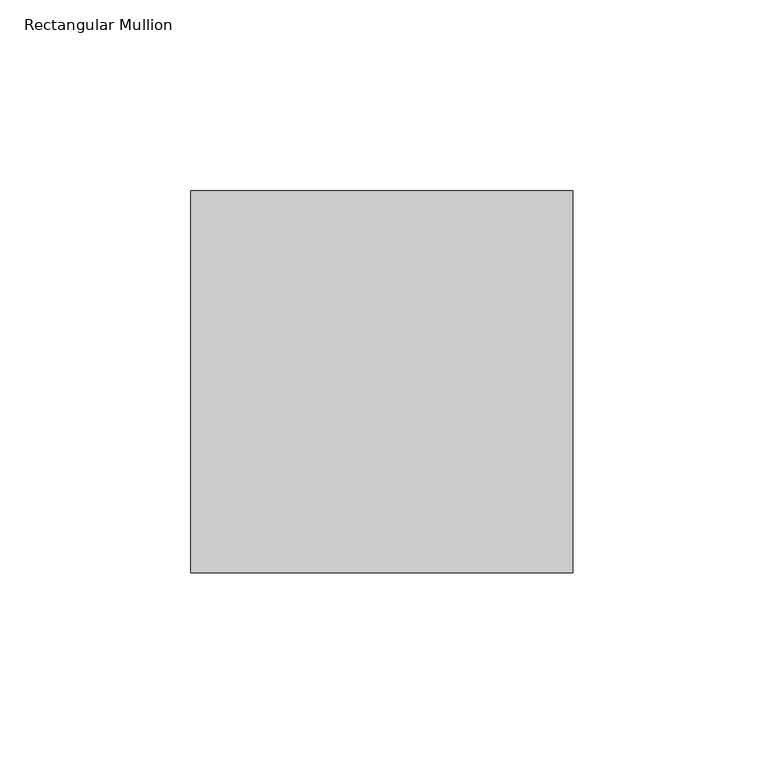
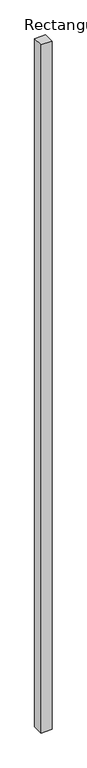
"""IFC4 building model written with IfcOpenShell, lengths in millimetres: member geometry, Rectangular Mullion : 알루미늄_Rectangular Cap_100 x100."""

import ifcopenshell
import ifcopenshell.guid

model = None  # the IFC model being written
_history = None  # IfcOwnerHistory: only IFC2X3 demands one
_inside = {}  # id of a spatial element -> (the spatial element, [elements in it])
_under = {}  # id of a project, library or spatial element -> (it, [spatial elements below it])
_declared = {}  # id of a project -> (the project, [libraries it declares])
_typed = {}  # id of a type object -> (the type object, [elements of that type])
_made_of = {}  # id of a material, layer set ... -> (it, [elements and type objects made of it])


def new_model(schema):
    """Start an empty IFC model of exactly this schema.

    Asked for "IFC4X3", IfcOpenShell would pick the latest addendum, in which some entities
    have other attributes; the version numbers below select the first issue.
    IFC2X3 requires an IfcOwnerHistory on every rooted entity: one is made here for all.
    """
    global model, _history
    if schema == "IFC4X3":
        model = ifcopenshell.file(schema_version=(4, 3, 0, 0))
    else:
        model = ifcopenshell.file(schema=schema)
    _inside.clear()
    _under.clear()
    _declared.clear()
    _typed.clear()
    _made_of.clear()
    _history = None
    if model.schema == "IFC2X3":
        org = make("IfcOrganization", Name="unknown")
        user = make(
            "IfcPersonAndOrganization",
            ThePerson=make("IfcPerson", FamilyName="unknown"),
            TheOrganization=org,
        )
        app = make(
            "IfcApplication",
            ApplicationDeveloper=org,
            Version="unknown",
            ApplicationFullName="unknown",
            ApplicationIdentifier="unknown",
        )
        _history = make(
            "IfcOwnerHistory",
            OwningUser=user,
            OwningApplication=app,
            ChangeAction="ADDED",
            CreationDate=0,
        )
    return model


def make(cls, **values):
    """One entity of the class cls with the attributes given. An attribute that is None is left unset."""
    return model.create_entity(
        cls, **{name: value for name, value in values.items() if value is not None}
    )


def rooted(cls, **values):
    """An entity with a GlobalId (a new one), such as an element, a storey or a relation."""
    return make(cls, GlobalId=ifcopenshell.guid.new(), OwnerHistory=_history, **values)


def si_unit(unit_type, name, prefix=None):
    """IfcSIUnit, for example si_unit("LENGTHUNIT", "METRE", prefix="MILLI")."""
    return make("IfcSIUnit", UnitType=unit_type, Prefix=prefix, Name=name)


def assignment(units):
    """IfcUnitAssignment: the units of a project."""
    return None if units is None else make("IfcUnitAssignment", Units=units)


def point(xyz):
    """IfcCartesianPoint."""
    return None if xyz is None else make("IfcCartesianPoint", Coordinates=xyz)


def direction(xyz):
    """IfcDirection."""
    return None if xyz is None else make("IfcDirection", DirectionRatios=xyz)


def frame(location, z_axis=None, x_axis=None):
    """IfcAxis2Placement3D, a coordinate frame: its origin and axes. An axis left out is left unset."""
    return make(
        "IfcAxis2Placement3D",
        Location=point(location),
        Axis=direction(z_axis),
        RefDirection=direction(x_axis),
    )


def origin():
    """The frame at (0, 0, 0) with its axes left unset."""
    return frame((0.0, 0.0, 0.0))


def place(relative_to, where):
    """IfcLocalPlacement: puts the frame where relative to a parent placement (None: the world)."""
    return make(
        "IfcLocalPlacement", PlacementRelTo=relative_to, RelativePlacement=where
    )


def context(
    kind, dimensions, precision=None, world=None, true_north=None, identifier=None
):
    """IfcGeometricRepresentationContext, for example the 3D "Model" context."""
    return make(
        "IfcGeometricRepresentationContext",
        ContextIdentifier=identifier,
        ContextType=kind,
        CoordinateSpaceDimension=dimensions,
        Precision=precision,
        WorldCoordinateSystem=world,
        TrueNorth=true_north,
    )


def project(units=None, contexts=None):
    """IfcProject with its units and contexts."""
    return rooted(
        "IfcProject",
        Name="project",
        RepresentationContexts=contexts,
        UnitsInContext=assignment(units),
    )


def spatial(cls, under=None, at=None, **own):
    """A site, building, storey or space (cls), placed at a placement, below another one or the project."""
    s = rooted(cls, ObjectPlacement=at, **own)
    if under is not None:
        _under.setdefault(under.id(), (under, []))[1].append(s)
    return s


def polyline(points):
    """IfcPolyline through the points."""
    return make("IfcPolyline", Points=[point(p) for p in points])


def outline(outer, holes=None, kind="AREA"):
    """IfcArbitraryClosedProfileDef: a profile drawn as a closed curve; with holes, ...WithVoids."""
    if holes is None:
        return make("IfcArbitraryClosedProfileDef", ProfileType=kind, OuterCurve=outer)
    return make(
        "IfcArbitraryProfileDefWithVoids",
        ProfileType=kind,
        OuterCurve=outer,
        InnerCurves=holes,
    )


def extrude(swept, where, along, depth):
    """IfcExtrudedAreaSolid: the profile swept, set in the frame where, extruded along a direction by depth."""
    return make(
        "IfcExtrudedAreaSolid",
        SweptArea=swept,
        Position=where,
        ExtrudedDirection=direction(along),
        Depth=depth,
    )


def shape(context_of_items, identifier, shape_type, items):
    """IfcShapeRepresentation: the items that make up one representation, for example the "Body"."""
    return make(
        "IfcShapeRepresentation",
        ContextOfItems=context_of_items,
        RepresentationIdentifier=identifier,
        RepresentationType=shape_type,
        Items=items,
    )


def source(mapping_origin, context_of_items, identifier, shape_type, items):
    """IfcRepresentationMap: a shape defined once, which mapped items show again and again."""
    return make(
        "IfcRepresentationMap",
        MappingOrigin=mapping_origin,
        MappedRepresentation=shape(context_of_items, identifier, shape_type, items),
    )


def transform(
    local_origin,
    x_axis=None,
    y_axis=None,
    z_axis=None,
    scale=None,
    scale2=None,
    scale3=None,
    uniform=True,
):
    """IfcCartesianTransformationOperator3D, or its non-uniform kind. x_axis, y_axis, z_axis: its Axis1, 2, 3."""
    if uniform:
        return make(
            "IfcCartesianTransformationOperator3D",
            Axis1=direction(x_axis),
            Axis2=direction(y_axis),
            LocalOrigin=point(local_origin),
            Scale=scale,
            Axis3=direction(z_axis),
        )
    return make(
        "IfcCartesianTransformationOperator3DnonUniform",
        Axis1=direction(x_axis),
        Axis2=direction(y_axis),
        LocalOrigin=point(local_origin),
        Scale=scale,
        Axis3=direction(z_axis),
        Scale2=scale2,
        Scale3=scale3,
    )


def mapped(mapping_source, mapping_target):
    """IfcMappedItem: shows the shape of a source again, moved by a transform."""
    return make(
        "IfcMappedItem", MappingSource=mapping_source, MappingTarget=mapping_target
    )


def made_of(thing, what):
    """Note that an element or type object is made of a material, layer set ...; save() writes the relation."""
    if what is not None:
        _made_of.setdefault(what.id(), (what, []))[1].append(thing)
    return thing


def element(
    cls,
    number,
    at=None,
    inside=None,
    cuts=None,
    type_object=None,
    material=None,
    context=None,
    identifier="Body",
    shape_type=None,
    held_by="IfcProductDefinitionShape",
    body=None,
    shapes=None,
    **own,
):
    """One element of the class cls, such as IfcWall. Its Tag is "e" and its number.

    at: its placement. inside: the storey or other place that contains it. cuts: it is an
    opening in that element (IfcRelVoidsElement). A single representation is given by context,
    identifier, shape_type and body (its items); several are given by shapes. held_by: the class
    of the entity that holds the representations. save() writes the other relations.
    """
    e = rooted(cls, Tag="e%d" % number, ObjectPlacement=at, **own)
    if body is not None:
        shapes = [shape(context, identifier, shape_type, body)]
    if shapes is not None:
        e.Representation = make(held_by, Representations=shapes)
    if inside is not None:
        _inside.setdefault(inside.id(), (inside, []))[1].append(e)
    if cuts is not None:
        rooted(
            "IfcRelVoidsElement", RelatingBuildingElement=cuts, RelatedOpeningElement=e
        )
    if type_object is not None:
        _typed.setdefault(type_object.id(), (type_object, []))[1].append(e)
    return made_of(e, material)


def aggregate(whole, parts):
    """IfcRelAggregates: a whole, such as a stair, and the parts it consists of."""
    return rooted("IfcRelAggregates", RelatingObject=whole, RelatedObjects=parts)


def save(model, path):
    """Write the relations noted so far, then the file.

    IfcRelAggregates (storeys below a building ...), IfcRelContainedInSpatialStructure (elements
    in a storey), IfcRelDefinesByType, IfcRelAssociatesMaterial and IfcRelDeclares: one each for
    every whole, place, type object, material and project.
    """
    for whole, parts in _under.values():
        aggregate(whole, parts)
    for where, things in _inside.values():
        rooted(
            "IfcRelContainedInSpatialStructure",
            RelatedElements=things,
            RelatingStructure=where,
        )
    for kind, things in _typed.values():
        rooted("IfcRelDefinesByType", RelatedObjects=things, RelatingType=kind)
    for what, things in _made_of.values():
        rooted("IfcRelAssociatesMaterial", RelatedObjects=things, RelatingMaterial=what)
    for by, libraries in _declared.values():
        rooted("IfcRelDeclares", RelatingContext=by, RelatedDefinitions=libraries)
    model.write(path)


def rectangular_mullion_46d195e2(model_context):
    return source(origin(), model_context, "Body", "SweptSolid", [
        extrude(outline(polyline([(0.0, 50.0), (0.0, -50.0), (-100.0, -50.0), (-100.0, 50.0), (0.0, 50.0)])), frame((0.0, 0.0, -6569.0), z_axis=(0.0, 0.0, 1.0), x_axis=(1.0, 0.0, 0.0)), (0.0, 0.0, 1.0), 6569.0),
    ])


if __name__ == "__main__":
    model = new_model("IFC4")
    model_context = context("Model", 3, world=origin())
    ifc_project = project(units=[si_unit("LENGTHUNIT", "METRE", prefix="MILLI")], contexts=[model_context])
    site = spatial("IfcSite", under=ifc_project)
    building = spatial("IfcBuilding", under=site)
    placement = place(None, origin())
    rectangular_mullion_shape = rectangular_mullion_46d195e2(model_context)
    element("IfcMember", 1, ObjectType="Rectangular Mullion : 알루미늄_Rectangular Cap_100 x100", at=placement, inside=building, context=model_context, shape_type="MappedRepresentation", body=[
        mapped(rectangular_mullion_shape, transform((0.0, 0.0, 0.0), x_axis=(1.0, 0.0, 0.0), y_axis=(0.0, 1.0, 0.0), z_axis=(0.0, 0.0, 1.0))),
    ])
    save(model, "model.ifc")

# Revit data of these elements
# Type "Rectangular Mullion : 알루미늄_Rectangular Cap_100 x100"
#   built-in parameter 1007304 = 0.328084 (stored number, unit not read)
#   built-in parameter 1007301 = 0.164042 (stored number, unit not read)
#   built-in parameter 1007300 = 0.164042 (stored number, unit not read)
# Element 1 (IfcMember, "Rectangular Mullion : 알루미늄_Rectangular Cap_100 x100")
#   Materials on its faces: "00_Metal_Stainless Steel"
# Materials
#   "00_Metal_Stainless Steel": class "Metal", colour RGB 148 148 148, transparency 0, Description = "Steel", Cost = 0
